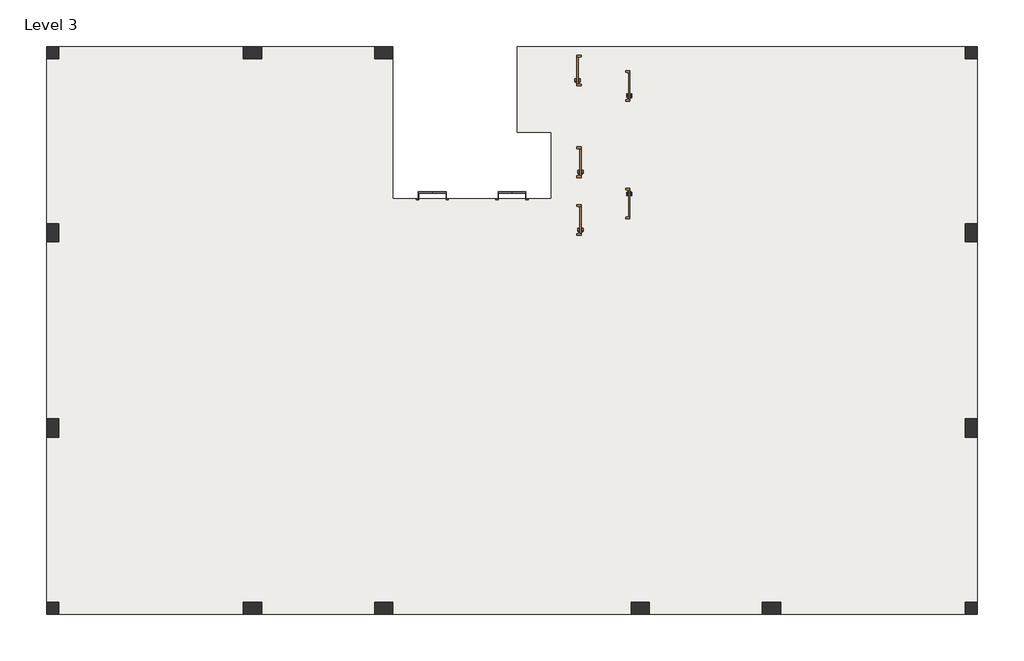
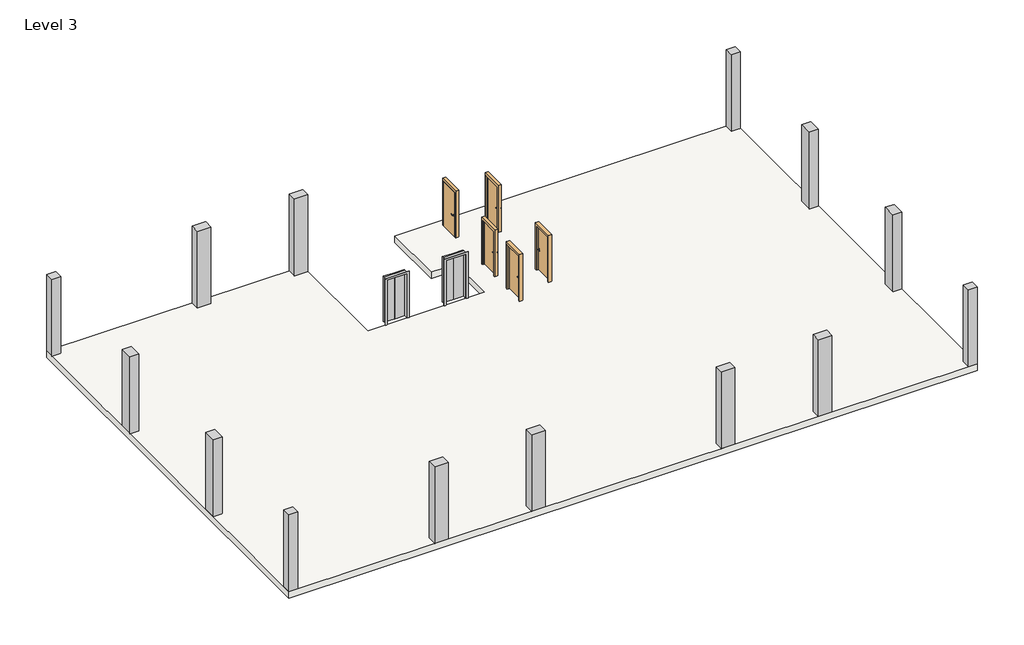
# One storey: 14 columns, 5 doors, 2 proxies, 1 slab.
"""IFC4 building model written with IfcOpenShell, lengths in millimetres."""

import ifcopenshell
import ifcopenshell.guid

model = None  # the IFC model being written
_history = None  # IfcOwnerHistory: only IFC2X3 demands one
_inside = {}  # id of a spatial element -> (the spatial element, [elements in it])
_under = {}  # id of a project, library or spatial element -> (it, [spatial elements below it])
_declared = {}  # id of a project -> (the project, [libraries it declares])
_typed = {}  # id of a type object -> (the type object, [elements of that type])
_made_of = {}  # id of a material, layer set ... -> (it, [elements and type objects made of it])


def new_model(schema):
    """Start an empty IFC model of exactly this schema.

    Asked for "IFC4X3", IfcOpenShell would pick the latest addendum, in which some entities
    have other attributes; the version numbers below select the first issue.
    IFC2X3 requires an IfcOwnerHistory on every rooted entity: one is made here for all.
    """
    global model, _history
    if schema == "IFC4X3":
        model = ifcopenshell.file(schema_version=(4, 3, 0, 0))
    else:
        model = ifcopenshell.file(schema=schema)
    _inside.clear()
    _under.clear()
    _declared.clear()
    _typed.clear()
    _made_of.clear()
    _history = None
    if model.schema == "IFC2X3":
        org = make("IfcOrganization", Name="unknown")
        user = make(
            "IfcPersonAndOrganization",
            ThePerson=make("IfcPerson", FamilyName="unknown"),
            TheOrganization=org,
        )
        app = make(
            "IfcApplication",
            ApplicationDeveloper=org,
            Version="unknown",
            ApplicationFullName="unknown",
            ApplicationIdentifier="unknown",
        )
        _history = make(
            "IfcOwnerHistory",
            OwningUser=user,
            OwningApplication=app,
            ChangeAction="ADDED",
            CreationDate=0,
        )
    return model


def make(cls, **values):
    """One entity of the class cls with the attributes given. An attribute that is None is left unset."""
    return model.create_entity(
        cls, **{name: value for name, value in values.items() if value is not None}
    )


def rooted(cls, **values):
    """An entity with a GlobalId (a new one), such as an element, a storey or a relation."""
    return make(cls, GlobalId=ifcopenshell.guid.new(), OwnerHistory=_history, **values)


def si_unit(unit_type, name, prefix=None):
    """IfcSIUnit, for example si_unit("LENGTHUNIT", "METRE", prefix="MILLI")."""
    return make("IfcSIUnit", UnitType=unit_type, Prefix=prefix, Name=name)


def assignment(units):
    """IfcUnitAssignment: the units of a project."""
    return None if units is None else make("IfcUnitAssignment", Units=units)


def point(xyz):
    """IfcCartesianPoint."""
    return None if xyz is None else make("IfcCartesianPoint", Coordinates=xyz)


def direction(xyz):
    """IfcDirection."""
    return None if xyz is None else make("IfcDirection", DirectionRatios=xyz)


def frame(location, z_axis=None, x_axis=None):
    """IfcAxis2Placement3D, a coordinate frame: its origin and axes. An axis left out is left unset."""
    return make(
        "IfcAxis2Placement3D",
        Location=point(location),
        Axis=direction(z_axis),
        RefDirection=direction(x_axis),
    )


def frame_2d(location, x_axis=None):
    """IfcAxis2Placement2D, a coordinate frame in the plane: its origin and x axis."""
    return make(
        "IfcAxis2Placement2D", Location=point(location), RefDirection=direction(x_axis)
    )


def origin():
    """The frame at (0, 0, 0) with its axes left unset."""
    return frame((0.0, 0.0, 0.0))


def origin_with_axes():
    """The frame at (0, 0, 0) with the z axis (0, 0, 1) and the x axis (1, 0, 0) written out."""
    return frame((0.0, 0.0, 0.0), z_axis=(0.0, 0.0, 1.0), x_axis=(1.0, 0.0, 0.0))


def place(relative_to, where):
    """IfcLocalPlacement: puts the frame where relative to a parent placement (None: the world)."""
    return make(
        "IfcLocalPlacement", PlacementRelTo=relative_to, RelativePlacement=where
    )


def context(
    kind, dimensions, precision=None, world=None, true_north=None, identifier=None
):
    """IfcGeometricRepresentationContext, for example the 3D "Model" context."""
    return make(
        "IfcGeometricRepresentationContext",
        ContextIdentifier=identifier,
        ContextType=kind,
        CoordinateSpaceDimension=dimensions,
        Precision=precision,
        WorldCoordinateSystem=world,
        TrueNorth=true_north,
    )


def project(units=None, contexts=None):
    """IfcProject with its units and contexts."""
    return rooted(
        "IfcProject",
        Name="project",
        RepresentationContexts=contexts,
        UnitsInContext=assignment(units),
    )


def spatial(cls, under=None, at=None, **own):
    """A site, building, storey or space (cls), placed at a placement, below another one or the project."""
    s = rooted(cls, ObjectPlacement=at, **own)
    if under is not None:
        _under.setdefault(under.id(), (under, []))[1].append(s)
    return s


def polyline(points):
    """IfcPolyline through the points."""
    return make("IfcPolyline", Points=[point(p) for p in points])


def circle_curve(where, radius):
    """IfcCircle in the frame where."""
    return make("IfcCircle", Position=where, Radius=radius)


def ellipse_curve(where, semi_axis1, semi_axis2):
    """IfcEllipse in the frame where."""
    return make(
        "IfcEllipse", Position=where, SemiAxis1=semi_axis1, SemiAxis2=semi_axis2
    )


def trimmed(basis, trim1, trim2, sense, master):
    """IfcTrimmedCurve: the piece of a basis curve between two trims."""
    return make(
        "IfcTrimmedCurve",
        BasisCurve=basis,
        Trim1=trim1,
        Trim2=trim2,
        SenseAgreement=sense,
        MasterRepresentation=master,
    )


def segment(curve, same_sense, transition):
    """IfcCompositeCurveSegment."""
    return make(
        "IfcCompositeCurveSegment",
        Transition=transition,
        SameSense=same_sense,
        ParentCurve=curve,
    )


def composite_curve(segments, self_intersect=None):
    """IfcCompositeCurve: segments joined end to end."""
    return make("IfcCompositeCurve", Segments=segments, SelfIntersect=self_intersect)


def outline(outer, holes=None, kind="AREA"):
    """IfcArbitraryClosedProfileDef: a profile drawn as a closed curve; with holes, ...WithVoids."""
    if holes is None:
        return make("IfcArbitraryClosedProfileDef", ProfileType=kind, OuterCurve=outer)
    return make(
        "IfcArbitraryProfileDefWithVoids",
        ProfileType=kind,
        OuterCurve=outer,
        InnerCurves=holes,
    )


def extrude(swept, where, along, depth):
    """IfcExtrudedAreaSolid: the profile swept, set in the frame where, extruded along a direction by depth."""
    return make(
        "IfcExtrudedAreaSolid",
        SweptArea=swept,
        Position=where,
        ExtrudedDirection=direction(along),
        Depth=depth,
    )


def faces_of(points, faces, orient=None, outer=None):
    """IfcFace entities. A face is a list of loops; a loop is a list of indices into points, from 0.

    orient and outer hold one flag for each loop. By default every Orientation is true, the
    first loop of a face is its IfcFaceOuterBound and the others are IfcFaceBound.
    """
    made = []
    for i, loops in enumerate(faces):
        bounds = []
        for j, loop in enumerate(loops):
            is_outer = j == 0 if outer is None else outer[i][j]
            bounds.append(
                make(
                    "IfcFaceOuterBound" if is_outer else "IfcFaceBound",
                    Bound=make("IfcPolyLoop", Polygon=[points[k] for k in loop]),
                    Orientation=True if orient is None else orient[i][j],
                )
            )
        made.append(make("IfcFace", Bounds=bounds))
    return made


def faceted_brep(points, faces, orient=None, outer=None, voids=None):
    """IfcFacetedBrep: a solid bounded by flat faces; with voids (closed shells), ...WithVoids."""
    shared = [point(p) for p in points]
    hull = make("IfcClosedShell", CfsFaces=faces_of(shared, faces, orient, outer))
    if voids is None:
        return make("IfcFacetedBrep", Outer=hull)
    return make(
        "IfcFacetedBrepWithVoids",
        Outer=hull,
        Voids=[
            make(cls, CfsFaces=faces_of(shared, fs, o, b)) for cls, fs, o, b in voids
        ],
    )


def shape(context_of_items, identifier, shape_type, items):
    """IfcShapeRepresentation: the items that make up one representation, for example the "Body"."""
    return make(
        "IfcShapeRepresentation",
        ContextOfItems=context_of_items,
        RepresentationIdentifier=identifier,
        RepresentationType=shape_type,
        Items=items,
    )


def source(mapping_origin, context_of_items, identifier, shape_type, items):
    """IfcRepresentationMap: a shape defined once, which mapped items show again and again."""
    return make(
        "IfcRepresentationMap",
        MappingOrigin=mapping_origin,
        MappedRepresentation=shape(context_of_items, identifier, shape_type, items),
    )


def transform(
    local_origin,
    x_axis=None,
    y_axis=None,
    z_axis=None,
    scale=None,
    scale2=None,
    scale3=None,
    uniform=True,
):
    """IfcCartesianTransformationOperator3D, or its non-uniform kind. x_axis, y_axis, z_axis: its Axis1, 2, 3."""
    if uniform:
        return make(
            "IfcCartesianTransformationOperator3D",
            Axis1=direction(x_axis),
            Axis2=direction(y_axis),
            LocalOrigin=point(local_origin),
            Scale=scale,
            Axis3=direction(z_axis),
        )
    return make(
        "IfcCartesianTransformationOperator3DnonUniform",
        Axis1=direction(x_axis),
        Axis2=direction(y_axis),
        LocalOrigin=point(local_origin),
        Scale=scale,
        Axis3=direction(z_axis),
        Scale2=scale2,
        Scale3=scale3,
    )


def mapped(mapping_source, mapping_target):
    """IfcMappedItem: shows the shape of a source again, moved by a transform."""
    return make(
        "IfcMappedItem", MappingSource=mapping_source, MappingTarget=mapping_target
    )


def made_of(thing, what):
    """Note that an element or type object is made of a material, layer set ...; save() writes the relation."""
    if what is not None:
        _made_of.setdefault(what.id(), (what, []))[1].append(thing)
    return thing


def element(
    cls,
    number,
    at=None,
    inside=None,
    cuts=None,
    type_object=None,
    material=None,
    context=None,
    identifier="Body",
    shape_type=None,
    held_by="IfcProductDefinitionShape",
    body=None,
    shapes=None,
    **own,
):
    """One element of the class cls, such as IfcWall. Its Tag is "e" and its number.

    at: its placement. inside: the storey or other place that contains it. cuts: it is an
    opening in that element (IfcRelVoidsElement). A single representation is given by context,
    identifier, shape_type and body (its items); several are given by shapes. held_by: the class
    of the entity that holds the representations. save() writes the other relations.
    """
    e = rooted(cls, Tag="e%d" % number, ObjectPlacement=at, **own)
    if body is not None:
        shapes = [shape(context, identifier, shape_type, body)]
    if shapes is not None:
        e.Representation = make(held_by, Representations=shapes)
    if inside is not None:
        _inside.setdefault(inside.id(), (inside, []))[1].append(e)
    if cuts is not None:
        rooted(
            "IfcRelVoidsElement", RelatingBuildingElement=cuts, RelatedOpeningElement=e
        )
    if type_object is not None:
        _typed.setdefault(type_object.id(), (type_object, []))[1].append(e)
    return made_of(e, material)


def aggregate(whole, parts):
    """IfcRelAggregates: a whole, such as a stair, and the parts it consists of."""
    return rooted("IfcRelAggregates", RelatingObject=whole, RelatedObjects=parts)


def save(model, path):
    """Write the relations noted so far, then the file.

    IfcRelAggregates (storeys below a building ...), IfcRelContainedInSpatialStructure (elements
    in a storey), IfcRelDefinesByType, IfcRelAssociatesMaterial and IfcRelDeclares: one each for
    every whole, place, type object, material and project.
    """
    for whole, parts in _under.values():
        aggregate(whole, parts)
    for where, things in _inside.values():
        rooted(
            "IfcRelContainedInSpatialStructure",
            RelatedElements=things,
            RelatingStructure=where,
        )
    for kind, things in _typed.values():
        rooted("IfcRelDefinesByType", RelatedObjects=things, RelatingType=kind)
    for what, things in _made_of.values():
        rooted("IfcRelAssociatesMaterial", RelatedObjects=things, RelatingMaterial=what)
    for by, libraries in _declared.values():
        rooted("IfcRelDeclares", RelatingContext=by, RelatedDefinitions=libraries)
    model.write(path)


def plane_surface(at):
    """IfcPlane: the flat surface through the origin of the frame at, square to its z axis."""
    return make("IfcPlane", Position=at)


def cylinder_surface(at, radius):
    """IfcCylindricalSurface: all points at the distance radius from the z axis of the frame at."""
    return make("IfcCylindricalSurface", Position=at, Radius=radius)


def revolved_surface(curve, axis_point, axis_direction):
    """IfcSurfaceOfRevolution: the curve turned about the line through axis_point along axis_direction."""
    return make(
        "IfcSurfaceOfRevolution",
        SweptCurve=make("IfcArbitraryOpenProfileDef", ProfileType="CURVE", Curve=curve),
        AxisPosition=make("IfcAxis1Placement", Location=point(axis_point), Axis=direction(axis_direction)),
    )


def advanced_brep(points, edges, surfaces, faces):
    """IfcAdvancedBrep: a solid bounded by faces that lie on surfaces and meet in shared edges.

    An edge is (start, end): straight between two places in points (the first is 0);
    or (start, end, curve); or (start, end, curve, False) where it runs against its curve.
    A face is (place in surfaces, loops), or (place, loops, False) where it looks against
    its surface's normal. A loop lists edges by number (the first is 1), with a minus sign
    where the edge is run from its end to its start. The first loop is the outer one.
    """
    corners = [point(p) for p in points]
    vertices = [make("IfcVertexPoint", VertexGeometry=c) for c in corners]
    made = []
    for start, end, *more in edges:
        made.append(
            make(
                "IfcEdgeCurve",
                EdgeStart=vertices[start],
                EdgeEnd=vertices[end],
                EdgeGeometry=more[0] if more else make("IfcPolyline", Points=[corners[start], corners[end]]),
                SameSense=more[1] if len(more) > 1 else True,
            )
        )
    hull = []
    for where, loops, *sense in faces:
        bounds = []
        for j, loop in enumerate(loops):
            ring = [make("IfcOrientedEdge", EdgeElement=made[abs(k) - 1], Orientation=k > 0) for k in loop]
            bounds.append(
                make(
                    "IfcFaceOuterBound" if j == 0 else "IfcFaceBound",
                    Bound=make("IfcEdgeLoop", EdgeList=ring),
                    Orientation=True,
                )
            )
        hull.append(make("IfcAdvancedFace", Bounds=bounds, FaceSurface=surfaces[where], SameSense=sense[0] if sense else True))
    return make("IfcAdvancedBrep", Outer=make("IfcClosedShell", CfsFaces=hull))


def proxy_71d7088b(model_context):
    return source(origin(), model_context, "Body", "SweptSolid", [
        extrude(outline(polyline([(-102.3106443, 96.8375), (-562.6856443, 96.8375), (-562.6856443, 147.6375), (-102.3106443, 147.6375), (-102.3106443, 96.8375)])), origin_with_axes(), (0.0, 0.0, 1.0), 2159.0),
        extrude(outline(polyline([(364.4143557, 96.8375), (-95.9606443, 96.8375), (-95.9606443, 147.6375), (364.4143557, 147.6375), (364.4143557, 96.8375)])), origin_with_axes(), (0.0, 0.0, 1.0), 2159.0),
        extrude(outline(polyline([(0.0, -562.6856443), (0.0, -556.3356443), (2133.6, -556.3356443), (2133.6, 358.0643557), (0.0, 358.0643557), (0.0, 364.4143557), (2159.0, 364.4143557), (2159.0, -562.6856443), (0.0, -562.6856443)])), frame((0.0, -96.8375, 0.0), z_axis=(0.0, 1.0, 0.0), x_axis=(0.0, 0.0, 1.0)), (0.0, 0.0, 1.0), 193.675),
        extrude(outline(polyline([(0.0, -632.5356443), (0.0, -556.3356443), (2133.6, -556.3356443), (2133.6, 358.0643557), (0.0, 358.0643557), (0.0, 434.2643557), (2209.8, 434.2643557), (2209.8, -632.5356443), (0.0, -632.5356443)])), frame((0.0, -122.2375, 0.0), z_axis=(0.0, 1.0, 0.0), x_axis=(0.0, 0.0, 1.0)), (0.0, 0.0, 1.0), 25.4),
    ])


def door_9f6fe377(model_context):
    return source(origin(), model_context, "Body", "SolidModel", [
        advanced_brep(
        [(-392.190625, -25.3375, 1016.0), (-372.190625, -25.3375, 1016.0), (-392.190625, 4.6625, 1016.0), (-372.190625, 4.6625, 1016.0), (-367.190625, 9.6625, 1016.0), (-367.190625, 29.6625, 1016.0), (-262.190625, 29.6625, 1016.0), (-262.190625, 9.6625, 1016.0)],
        [
            (0, 1, circle_curve(frame((-382.190625, -25.3375, 1016.0), z_axis=(0.0, -1.0, 0.0), x_axis=(1.0, 0.0, 0.0)), 10.0)),
            (1, 0, circle_curve(frame((-382.190625, -25.3375, 1016.0), z_axis=(0.0, -1.0, 0.0), x_axis=(1.0, 0.0, 0.0)), 10.0)),
            (0, 2),
            (2, 3, circle_curve(frame((-382.190625, 4.6625, 1016.0), z_axis=(0.0, -1.0, 0.0), x_axis=(1.0, 0.0, 0.0)), 10.0)),
            (3, 1),
            (3, 2, circle_curve(frame((-382.190625, 4.6625, 1016.0), z_axis=(0.0, -1.0, 0.0), x_axis=(1.0, 0.0, 0.0)), 10.0)),
            (4, 3, circle_curve(frame((-367.190625, 4.6625, 1016.0), z_axis=(0.0, 0.0, 1.0), x_axis=(-1.0, 0.0, 0.0)), 5.0)),
            (2, 5, circle_curve(frame((-367.190625, 4.6625, 1016.0), z_axis=(0.0, 0.0, -1.0), x_axis=(-1.0, 0.0, 0.0)), 25.0)),
            (5, 4, circle_curve(frame((-367.190625, 19.6625, 1016.0), z_axis=(-1.0, 0.0, 0.0), x_axis=(0.0, -1.0, 0.0)), 10.0)),
            (4, 5, circle_curve(frame((-367.190625, 19.6625, 1016.0), z_axis=(-1.0, 0.0, 0.0), x_axis=(0.0, -1.0, 0.0)), 10.0)),
            (6, 7, circle_curve(frame((-262.190625, 19.6625, 1016.0), z_axis=(1.0, 0.0, 0.0), x_axis=(0.0, -1.0, 0.0)), 10.0)),
            (7, 6, circle_curve(frame((-262.190625, 19.6625, 1016.0), z_axis=(1.0, 0.0, 0.0), x_axis=(0.0, -1.0, 0.0)), 10.0)),
            (5, 6),
            (7, 4),
        ],
        [
            plane_surface(frame((-382.190625, -25.3375, 1016.0), z_axis=(0.0, -1.0, 0.0), x_axis=(0.0, 0.0, 1.0))),
            cylinder_surface(frame((-382.190625, -25.3375, 1016.0), z_axis=(0.0, -1.0, 0.0), x_axis=(1.0, 0.0, 0.0)), 10.0),
            revolved_surface(trimmed(ellipse_curve(frame((-382.190625, 4.6625, 1016.0), z_axis=(0.0, -1.0, 0.0), x_axis=(1.0, 0.0, 0.0)), 10.0, 10.0), [point((-392.190625, 4.6625, 1016.0))], [point((-372.190625, 4.6625, 1016.0))], True, "CARTESIAN"), (-367.190625, 4.6625, 1016.0), (0.0, 0.0, -1.0)),
            revolved_surface(trimmed(ellipse_curve(frame((-382.190625, 4.6625, 1016.0), z_axis=(0.0, -1.0, 0.0), x_axis=(1.0, 0.0, 0.0)), 10.0, 10.0), [point((-372.190625, 4.6625, 1016.0))], [point((-392.190625, 4.6625, 1016.0))], True, "CARTESIAN"), (-367.190625, 4.6625, 1016.0), (0.0, 0.0, -1.0)),
            plane_surface(frame((-262.190625, 19.6625, 1016.0), z_axis=(1.0, 0.0, 0.0), x_axis=(0.0, 0.0, 1.0))),
            cylinder_surface(frame((-367.190625, 19.6625, 1016.0), z_axis=(-1.0, 0.0, 0.0), x_axis=(0.0, -1.0, 0.0)), 10.0),
        ],
        [
            (0, [[1, 2]]),
            (1, [[-1, 3, 4, 5]]),
            (1, [[-2, -5, 6, -3]]),
            (2, [[7, -4, 8, 9]]),
            (3, [[-8, -6, -7, 10]]),
            (4, [[11, 12]]),
            (5, [[-9, 13, -12, 14]]),
            (5, [[-10, -14, -11, -13]]),
        ],
    ),
        extrude(outline(composite_curve([segment(trimmed(circle_curve(frame_2d((1016.0, -384.690625)), 30.0), [point((1016.0, -414.690625))], [point((1016.0, -354.690625))], False, "CARTESIAN"), True, "CONTINUOUS"), segment(trimmed(circle_curve(frame_2d((1016.0, -384.690625)), 30.0), [point((1016.0, -354.690625))], [point((1016.0, -414.690625))], False, "CARTESIAN"), True, "CONTINUOUS")], self_intersect=False)), frame((0.0, -33.3375, 0.0), z_axis=(0.0, 1.0, 0.0), x_axis=(0.0, 0.0, 1.0)), (0.0, 0.0, 1.0), 8.0),
        advanced_brep(
        [(-392.190625, -85.7875, 1016.0), (-372.190625, -85.7875, 1016.0), (-372.190625, -115.7875, 1016.0), (-392.190625, -115.7875, 1016.0), (-367.190625, -120.7875, 1016.0), (-367.190625, -140.7875, 1016.0), (-262.190625, -140.7875, 1016.0), (-262.190625, -120.7875, 1016.0)],
        [
            (0, 1, circle_curve(frame((-382.190625, -85.7875, 1016.0), z_axis=(0.0, 1.0, 0.0), x_axis=(1.0, 0.0, 0.0)), 10.0)),
            (1, 0, circle_curve(frame((-382.190625, -85.7875, 1016.0), z_axis=(0.0, 1.0, 0.0), x_axis=(1.0, 0.0, 0.0)), 10.0)),
            (1, 2),
            (2, 3, circle_curve(frame((-382.190625, -115.7875, 1016.0), z_axis=(0.0, 1.0, 0.0), x_axis=(1.0, 0.0, 0.0)), 10.0)),
            (3, 0),
            (3, 2, circle_curve(frame((-382.190625, -115.7875, 1016.0), z_axis=(0.0, 1.0, 0.0), x_axis=(1.0, 0.0, 0.0)), 10.0)),
            (4, 5, circle_curve(frame((-367.190625, -130.7875, 1016.0), z_axis=(-1.0, 0.0, 0.0), x_axis=(0.0, 1.0, 0.0)), 10.0)),
            (5, 3, circle_curve(frame((-367.190625, -115.7875, 1016.0), z_axis=(0.0, 0.0, -1.0), x_axis=(-1.0, 0.0, 0.0)), 25.0)),
            (2, 4, circle_curve(frame((-367.190625, -115.7875, 1016.0), z_axis=(0.0, 0.0, 1.0), x_axis=(-1.0, 0.0, 0.0)), 5.0)),
            (5, 4, circle_curve(frame((-367.190625, -130.7875, 1016.0), z_axis=(-1.0, 0.0, 0.0), x_axis=(0.0, 1.0, 0.0)), 10.0)),
            (6, 7, circle_curve(frame((-262.190625, -130.7875, 1016.0), z_axis=(1.0, 0.0, 0.0), x_axis=(0.0, 1.0, 0.0)), 10.0)),
            (7, 6, circle_curve(frame((-262.190625, -130.7875, 1016.0), z_axis=(1.0, 0.0, 0.0), x_axis=(0.0, 1.0, 0.0)), 10.0)),
            (4, 7),
            (6, 5),
        ],
        [
            plane_surface(frame((-382.190625, -85.7875, 1016.0), z_axis=(0.0, 1.0, 0.0), x_axis=(0.0, 0.0, 1.0))),
            cylinder_surface(frame((-382.190625, -85.7875, 1016.0), z_axis=(0.0, 1.0, 0.0), x_axis=(1.0, 0.0, 0.0)), 10.0),
            revolved_surface(trimmed(ellipse_curve(frame((-382.190625, -115.7875, 1016.0), z_axis=(0.0, -1.0, 0.0), x_axis=(1.0, 0.0, 0.0)), 10.0, 10.0), [point((-392.190625, -115.7875, 1016.0))], [point((-372.190625, -115.7875, 1016.0))], True, "CARTESIAN"), (-367.190625, -115.7875, 1016.0), (0.0, 0.0, -1.0)),
            revolved_surface(trimmed(ellipse_curve(frame((-382.190625, -115.7875, 1016.0), z_axis=(0.0, -1.0, 0.0), x_axis=(1.0, 0.0, 0.0)), 10.0, 10.0), [point((-372.190625, -115.7875, 1016.0))], [point((-392.190625, -115.7875, 1016.0))], True, "CARTESIAN"), (-367.190625, -115.7875, 1016.0), (0.0, 0.0, -1.0)),
            plane_surface(frame((-262.190625, -130.7875, 1016.0), z_axis=(1.0, 0.0, 0.0), x_axis=(0.0, 0.0, 1.0))),
            cylinder_surface(frame((-367.190625, -130.7875, 1016.0), z_axis=(-1.0, 0.0, 0.0), x_axis=(0.0, 1.0, 0.0)), 10.0),
        ],
        [
            (0, [[1, 2]]),
            (1, [[3, 4, 5, -2]]),
            (1, [[-5, 6, -3, -1]]),
            (2, [[7, 8, -4, 9]]),
            (3, [[10, -9, -6, -8]]),
            (4, [[11, 12]]),
            (5, [[13, -11, 14, -7]]),
            (5, [[-14, -12, -13, -10]]),
        ],
    ),
        extrude(outline(composite_curve([segment(trimmed(circle_curve(frame_2d((1016.0, -384.690625)), 30.0), [point((1016.0, -414.690625))], [point((1016.0, -354.690625))], False, "CARTESIAN"), True, "CONTINUOUS"), segment(trimmed(circle_curve(frame_2d((1016.0, -384.690625)), 30.0), [point((1016.0, -354.690625))], [point((1016.0, -414.690625))], False, "CARTESIAN"), True, "CONTINUOUS")], self_intersect=False)), frame((0.0, -85.7875, 0.0), z_axis=(0.0, 1.0, 0.0), x_axis=(0.0, 0.0, 1.0)), (0.0, 0.0, 1.0), 8.0),
        faceted_brep([(457.2, -28.575, 0.0), (441.325, -28.575, 0.0), (441.325, 19.05, 0.0), (457.2, 19.05, 0.0), (457.2, 68.2625, 0.0), (508.0, 68.2625, 0.0), (508.0, -77.7875, 0.0), (457.2, -77.7875, 0.0), (457.2, -77.7875, 2133.6), (457.2, -28.575, 2133.6), (508.0, -77.7875, 2235.2), (-508.0, -77.7875, 2235.2), (-508.0, -77.7875, 0.0), (-457.2, -77.7875, 0.0), (-457.2, -77.7875, 2133.6), (508.0, 68.2625, 2235.2), (457.2, 68.2625, 2133.6), (-457.2, 68.2625, 2133.6), (-457.2, 68.2625, 0.0), (-508.0, 68.2625, 0.0), (-508.0, 68.2625, 2235.2), (457.2, 19.05, 2133.6), (441.325, 19.05, 2117.725), (-441.325, 19.05, 2117.725), (-441.325, 19.05, 0.0), (-457.2, 19.05, 0.0), (-457.2, 19.05, 2133.6), (441.325, -28.575, 2117.725), (-457.2, -28.575, 2133.6), (-457.2, -28.575, 0.0), (-441.325, -28.575, 0.0), (-441.325, -28.575, 2117.725)], [[[0, 1, 2, 3, 4, 5, 6, 7]], [[7, 8, 9, 0]], [[6, 10, 11, 12, 13, 14, 8, 7]], [[5, 15, 10, 6]], [[4, 16, 17, 18, 19, 20, 15, 5]], [[3, 21, 16, 4]], [[2, 22, 23, 24, 25, 26, 21, 3]], [[1, 27, 22, 2]], [[0, 9, 28, 29, 30, 31, 27, 1]], [[8, 14, 28, 9]], [[16, 21, 26, 17]], [[22, 27, 31, 23]], [[12, 19, 18, 25, 24, 30, 29, 13]], [[13, 29, 28, 14]], [[11, 20, 19, 12]], [[17, 26, 25, 18]], [[23, 31, 30, 24]], [[15, 20, 11, 10]]]),
        extrude(outline(polyline([(457.2, -33.3375), (457.2, -77.7875), (-457.2, -77.7875), (-457.2, -33.3375), (457.2, -33.3375)])), origin_with_axes(), (0.0, 0.0, 1.0), 2133.6),
    ])


def door_87fe937e(model_context):
    return source(origin(), model_context, "Body", "SolidModel", [
        advanced_brep(
        [(-392.190625, 25.3375, 1016.0), (-372.190625, 25.3375, 1016.0), (-372.190625, -4.6625, 1016.0), (-392.190625, -4.6625, 1016.0), (-367.190625, -9.6625, 1016.0), (-367.190625, -29.6625, 1016.0), (-262.190625, -29.6625, 1016.0), (-262.190625, -9.6625, 1016.0)],
        [
            (0, 1, circle_curve(frame((-382.190625, 25.3375, 1016.0), z_axis=(0.0, 1.0, 0.0), x_axis=(1.0, 0.0, 0.0)), 10.0)),
            (1, 0, circle_curve(frame((-382.190625, 25.3375, 1016.0), z_axis=(0.0, 1.0, 0.0), x_axis=(1.0, 0.0, 0.0)), 10.0)),
            (1, 2),
            (2, 3, circle_curve(frame((-382.190625, -4.6625, 1016.0), z_axis=(0.0, 1.0, 0.0), x_axis=(1.0, 0.0, 0.0)), 10.0)),
            (3, 0),
            (3, 2, circle_curve(frame((-382.190625, -4.6625, 1016.0), z_axis=(0.0, 1.0, 0.0), x_axis=(1.0, 0.0, 0.0)), 10.0)),
            (4, 5, circle_curve(frame((-367.190625, -19.6625, 1016.0), z_axis=(-1.0, 0.0, 0.0), x_axis=(0.0, 1.0, 0.0)), 10.0)),
            (5, 3, circle_curve(frame((-367.190625, -4.6625, 1016.0), z_axis=(0.0, 0.0, -1.0), x_axis=(-1.0, 0.0, 0.0)), 25.0)),
            (2, 4, circle_curve(frame((-367.190625, -4.6625, 1016.0), z_axis=(0.0, 0.0, 1.0), x_axis=(-1.0, 0.0, 0.0)), 5.0)),
            (5, 4, circle_curve(frame((-367.190625, -19.6625, 1016.0), z_axis=(-1.0, 0.0, 0.0), x_axis=(0.0, 1.0, 0.0)), 10.0)),
            (6, 7, circle_curve(frame((-262.190625, -19.6625, 1016.0), z_axis=(1.0, 0.0, 0.0), x_axis=(0.0, 1.0, 0.0)), 10.0)),
            (7, 6, circle_curve(frame((-262.190625, -19.6625, 1016.0), z_axis=(1.0, 0.0, 0.0), x_axis=(0.0, 1.0, 0.0)), 10.0)),
            (4, 7),
            (6, 5),
        ],
        [
            plane_surface(frame((-382.190625, 25.3375, 1016.0), z_axis=(0.0, 1.0, 0.0), x_axis=(0.0, 0.0, 1.0))),
            cylinder_surface(frame((-382.190625, 25.3375, 1016.0), z_axis=(0.0, 1.0, 0.0), x_axis=(1.0, 0.0, 0.0)), 10.0),
            revolved_surface(trimmed(ellipse_curve(frame((-382.190625, -4.6625, 1016.0), z_axis=(0.0, -1.0, 0.0), x_axis=(1.0, 0.0, 0.0)), 10.0, 10.0), [point((-392.190625, -4.6625, 1016.0))], [point((-372.190625, -4.6625, 1016.0))], True, "CARTESIAN"), (-367.190625, -4.6625, 1016.0), (0.0, 0.0, -1.0)),
            revolved_surface(trimmed(ellipse_curve(frame((-382.190625, -4.6625, 1016.0), z_axis=(0.0, -1.0, 0.0), x_axis=(1.0, 0.0, 0.0)), 10.0, 10.0), [point((-372.190625, -4.6625, 1016.0))], [point((-392.190625, -4.6625, 1016.0))], True, "CARTESIAN"), (-367.190625, -4.6625, 1016.0), (0.0, 0.0, -1.0)),
            plane_surface(frame((-262.190625, -19.6625, 1016.0), z_axis=(1.0, 0.0, 0.0), x_axis=(0.0, 0.0, 1.0))),
            cylinder_surface(frame((-367.190625, -19.6625, 1016.0), z_axis=(-1.0, 0.0, 0.0), x_axis=(0.0, 1.0, 0.0)), 10.0),
        ],
        [
            (0, [[1, 2]]),
            (1, [[3, 4, 5, -2]]),
            (1, [[-5, 6, -3, -1]]),
            (2, [[7, 8, -4, 9]]),
            (3, [[10, -9, -6, -8]]),
            (4, [[11, 12]]),
            (5, [[13, -11, 14, -7]]),
            (5, [[-14, -12, -13, -10]]),
        ],
    ),
        extrude(outline(composite_curve([segment(trimmed(circle_curve(frame_2d((1016.0, -384.690625)), 30.0), [point((1016.0, -414.690625))], [point((1016.0, -354.690625))], False, "CARTESIAN"), True, "CONTINUOUS"), segment(trimmed(circle_curve(frame_2d((1016.0, -384.690625)), 30.0), [point((1016.0, -354.690625))], [point((1016.0, -414.690625))], False, "CARTESIAN"), True, "CONTINUOUS")], self_intersect=False)), frame((0.0, 25.3375, 0.0), z_axis=(0.0, 1.0, 0.0), x_axis=(0.0, 0.0, 1.0)), (0.0, 0.0, 1.0), 8.0),
        advanced_brep(
        [(-392.190625, 85.7875, 1016.0), (-372.190625, 85.7875, 1016.0), (-392.190625, 115.7875, 1016.0), (-372.190625, 115.7875, 1016.0), (-367.190625, 120.7875, 1016.0), (-367.190625, 140.7875, 1016.0), (-262.190625, 140.7875, 1016.0), (-262.190625, 120.7875, 1016.0)],
        [
            (0, 1, circle_curve(frame((-382.190625, 85.7875, 1016.0), z_axis=(0.0, -1.0, 0.0), x_axis=(1.0, 0.0, 0.0)), 10.0)),
            (1, 0, circle_curve(frame((-382.190625, 85.7875, 1016.0), z_axis=(0.0, -1.0, 0.0), x_axis=(1.0, 0.0, 0.0)), 10.0)),
            (0, 2),
            (2, 3, circle_curve(frame((-382.190625, 115.7875, 1016.0), z_axis=(0.0, -1.0, 0.0), x_axis=(1.0, 0.0, 0.0)), 10.0)),
            (3, 1),
            (3, 2, circle_curve(frame((-382.190625, 115.7875, 1016.0), z_axis=(0.0, -1.0, 0.0), x_axis=(1.0, 0.0, 0.0)), 10.0)),
            (4, 3, circle_curve(frame((-367.190625, 115.7875, 1016.0), z_axis=(0.0, 0.0, 1.0), x_axis=(-1.0, 0.0, 0.0)), 5.0)),
            (2, 5, circle_curve(frame((-367.190625, 115.7875, 1016.0), z_axis=(0.0, 0.0, -1.0), x_axis=(-1.0, 0.0, 0.0)), 25.0)),
            (5, 4, circle_curve(frame((-367.190625, 130.7875, 1016.0), z_axis=(-1.0, 0.0, 0.0), x_axis=(0.0, -1.0, 0.0)), 10.0)),
            (4, 5, circle_curve(frame((-367.190625, 130.7875, 1016.0), z_axis=(-1.0, 0.0, 0.0), x_axis=(0.0, -1.0, 0.0)), 10.0)),
            (6, 7, circle_curve(frame((-262.190625, 130.7875, 1016.0), z_axis=(1.0, 0.0, 0.0), x_axis=(0.0, -1.0, 0.0)), 10.0)),
            (7, 6, circle_curve(frame((-262.190625, 130.7875, 1016.0), z_axis=(1.0, 0.0, 0.0), x_axis=(0.0, -1.0, 0.0)), 10.0)),
            (5, 6),
            (7, 4),
        ],
        [
            plane_surface(frame((-382.190625, 85.7875, 1016.0), z_axis=(0.0, -1.0, 0.0), x_axis=(0.0, 0.0, 1.0))),
            cylinder_surface(frame((-382.190625, 85.7875, 1016.0), z_axis=(0.0, -1.0, 0.0), x_axis=(1.0, 0.0, 0.0)), 10.0),
            revolved_surface(trimmed(ellipse_curve(frame((-382.190625, 115.7875, 1016.0), z_axis=(0.0, -1.0, 0.0), x_axis=(1.0, 0.0, 0.0)), 10.0, 10.0), [point((-392.190625, 115.7875, 1016.0))], [point((-372.190625, 115.7875, 1016.0))], True, "CARTESIAN"), (-367.190625, 115.7875, 1016.0), (0.0, 0.0, -1.0)),
            revolved_surface(trimmed(ellipse_curve(frame((-382.190625, 115.7875, 1016.0), z_axis=(0.0, -1.0, 0.0), x_axis=(1.0, 0.0, 0.0)), 10.0, 10.0), [point((-372.190625, 115.7875, 1016.0))], [point((-392.190625, 115.7875, 1016.0))], True, "CARTESIAN"), (-367.190625, 115.7875, 1016.0), (0.0, 0.0, -1.0)),
            plane_surface(frame((-262.190625, 130.7875, 1016.0), z_axis=(1.0, 0.0, 0.0), x_axis=(0.0, 0.0, 1.0))),
            cylinder_surface(frame((-367.190625, 130.7875, 1016.0), z_axis=(-1.0, 0.0, 0.0), x_axis=(0.0, -1.0, 0.0)), 10.0),
        ],
        [
            (0, [[1, 2]]),
            (1, [[-1, 3, 4, 5]]),
            (1, [[-2, -5, 6, -3]]),
            (2, [[7, -4, 8, 9]]),
            (3, [[-8, -6, -7, 10]]),
            (4, [[11, 12]]),
            (5, [[-9, 13, -12, 14]]),
            (5, [[-10, -14, -11, -13]]),
        ],
    ),
        extrude(outline(composite_curve([segment(trimmed(circle_curve(frame_2d((1016.0, -384.690625)), 30.0), [point((1016.0, -414.690625))], [point((1016.0, -354.690625))], False, "CARTESIAN"), True, "CONTINUOUS"), segment(trimmed(circle_curve(frame_2d((1016.0, -384.690625)), 30.0), [point((1016.0, -354.690625))], [point((1016.0, -414.690625))], False, "CARTESIAN"), True, "CONTINUOUS")], self_intersect=False)), frame((0.0, 77.7875, 0.0), z_axis=(0.0, 1.0, 0.0), x_axis=(0.0, 0.0, 1.0)), (0.0, 0.0, 1.0), 8.0),
        faceted_brep([(457.2, 28.575, 0.0), (457.2, 77.7875, 0.0), (508.0, 77.7875, 0.0), (508.0, -68.2625, 0.0), (457.2, -68.2625, 0.0), (457.2, -19.05, 0.0), (441.325, -19.05, 0.0), (441.325, 28.575, 0.0), (457.2, 28.575, 2133.6), (457.2, 77.7875, 2133.6), (-457.2, 77.7875, 2133.6), (-457.2, 77.7875, 0.0), (-508.0, 77.7875, 0.0), (-508.0, 77.7875, 2235.2), (508.0, 77.7875, 2235.2), (508.0, -68.2625, 2235.2), (-508.0, -68.2625, 2235.2), (-508.0, -68.2625, 0.0), (-457.2, -68.2625, 0.0), (-457.2, -68.2625, 2133.6), (457.2, -68.2625, 2133.6), (457.2, -19.05, 2133.6), (-457.2, -19.05, 2133.6), (-457.2, -19.05, 0.0), (-441.325, -19.05, 0.0), (-441.325, -19.05, 2117.725), (441.325, -19.05, 2117.725), (441.325, 28.575, 2117.725), (-441.325, 28.575, 2117.725), (-441.325, 28.575, 0.0), (-457.2, 28.575, 0.0), (-457.2, 28.575, 2133.6)], [[[0, 1, 2, 3, 4, 5, 6, 7]], [[1, 0, 8, 9]], [[2, 1, 9, 10, 11, 12, 13, 14]], [[3, 2, 14, 15]], [[4, 3, 15, 16, 17, 18, 19, 20]], [[5, 4, 20, 21]], [[6, 5, 21, 22, 23, 24, 25, 26]], [[7, 6, 26, 27]], [[0, 7, 27, 28, 29, 30, 31, 8]], [[9, 8, 31, 10]], [[20, 19, 22, 21]], [[26, 25, 28, 27]], [[12, 11, 30, 29, 24, 23, 18, 17]], [[11, 10, 31, 30]], [[13, 12, 17, 16]], [[19, 18, 23, 22]], [[25, 24, 29, 28]], [[15, 14, 13, 16]]]),
        extrude(outline(polyline([(457.2, 33.3375), (-457.2, 33.3375), (-457.2, 77.7875), (457.2, 77.7875), (457.2, 33.3375)])), origin_with_axes(), (0.0, 0.0, 1.0), 2133.6),
    ])


model = new_model("IFC4")

# Units and contexts
model_context = context("Model", 3, world=origin())
ifc_project = project(units=[si_unit("LENGTHUNIT", "METRE", prefix="MILLI")], contexts=[model_context])

# Site, building, storey
site = spatial("IfcSite", under=ifc_project)
building = spatial("IfcBuilding", under=site)
storey = spatial("IfcBuildingStorey", under=building, Name="Level 3", Elevation=7315.2)

# Proxies
placement = place(None, origin())
proxy_shape = proxy_71d7088b(model_context)
element("IfcBuildingElementProxy", 1, Name="Elevator Door-Center : 36\" x 84\"", ObjectType="Elevator Door-Center : 36\" x 84\"", at=placement, inside=storey, context=model_context, shape_type="MappedRepresentation", body=[
    mapped(proxy_shape, transform((-3717.8016289, 4317.8640304, 7315.2), x_axis=(1.0, 0.0, 0.0), y_axis=(0.0, 1.0, 0.0), z_axis=(0.0, 0.0, 1.0))),
])
element("IfcBuildingElementProxy", 2, Name="Elevator Door-Center : 36\" x 84\"", ObjectType="Elevator Door-Center : 36\" x 84\"", at=placement, inside=storey, context=model_context, shape_type="MappedRepresentation", body=[
    mapped(proxy_shape, transform((-1066.6766289, 4317.8640304, 7315.2), x_axis=(1.0, 0.0, 0.0), y_axis=(0.0, 1.0, 0.0), z_axis=(0.0, 0.0, 1.0))),
])

# Columns
element("IfcColumn", 3, ObjectType="Rectangular Column : 24\" x 24\"", at=placement, inside=storey, context=model_context, shape_type="SweptSolid", body=[
    extrude(outline(polyline([(-16253.4122732, 9291.5015304), (-16253.4122732, 8885.1015304), (-16659.8122732, 8885.1015304), (-16659.8122732, 9291.5015304), (-16253.4122732, 9291.5015304)])), frame((0.0, 0.0, 7315.2), z_axis=(0.0, 0.0, 1.0), x_axis=(1.0, 0.0, 0.0)), (0.0, 0.0, 1.0), 3657.6),
])
element("IfcColumn", 4, ObjectType="Rectangular Column : 24\" x 24\"", at=placement, inside=storey, context=model_context, shape_type="SweptSolid", body=[
    extrude(outline(polyline([(-16253.4122732, 3398.7015304), (-16253.4122732, 2789.1015304), (-16659.8122732, 2789.1015304), (-16659.8122732, 3398.7015304), (-16253.4122732, 3398.7015304)])), frame((0.0, 0.0, 7315.2), z_axis=(0.0, 0.0, 1.0), x_axis=(1.0, 0.0, 0.0)), (0.0, 0.0, 1.0), 3657.6),
])
element("IfcColumn", 5, ObjectType="Rectangular Column : 24\" x 24\"", at=placement, inside=storey, context=model_context, shape_type="SweptSolid", body=[
    extrude(outline(polyline([(-9497.0122732, 8885.1015304), (-10106.6122732, 8885.1015304), (-10106.6122732, 9291.5015304), (-9497.0122732, 9291.5015304), (-9497.0122732, 8885.1015304)])), frame((0.0, 0.0, 7315.2), z_axis=(0.0, 0.0, 1.0), x_axis=(1.0, 0.0, 0.0)), (0.0, 0.0, 1.0), 3657.6),
])
element("IfcColumn", 6, ObjectType="Rectangular Column : 24\" x 24\"", at=placement, inside=storey, context=model_context, shape_type="SweptSolid", body=[
    extrude(outline(polyline([(-5128.2122732, 8885.1015304), (-5737.8122732, 8885.1015304), (-5737.8122732, 9291.5015304), (-5128.2122732, 9291.5015304), (-5128.2122732, 8885.1015304)])), frame((0.0, 0.0, 7315.2), z_axis=(0.0, 0.0, 1.0), x_axis=(1.0, 0.0, 0.0)), (0.0, 0.0, 1.0), 3657.6),
])
element("IfcColumn", 7, ObjectType="Rectangular Column : 24\" x 24\"", at=placement, inside=storey, context=model_context, shape_type="SweptSolid", body=[
    extrude(outline(polyline([(14328.1877268, 8885.1015304), (13921.7877268, 8885.1015304), (13921.7877268, 9291.5015304), (14328.1877268, 9291.5015304), (14328.1877268, 8885.1015304)])), frame((0.0, 0.0, 7315.2), z_axis=(0.0, 0.0, 1.0), x_axis=(1.0, 0.0, 0.0)), (0.0, 0.0, 1.0), 3657.6),
])
element("IfcColumn", 8, ObjectType="Rectangular Column : 24\" x 24\"", at=placement, inside=storey, context=model_context, shape_type="SweptSolid", body=[
    extrude(outline(polyline([(13921.7877268, 2789.1015304), (13921.7877268, 3398.7015304), (14328.1877268, 3398.7015304), (14328.1877268, 2789.1015304), (13921.7877268, 2789.1015304)])), frame((0.0, 0.0, 7315.2), z_axis=(0.0, 0.0, 1.0), x_axis=(1.0, 0.0, 0.0)), (0.0, 0.0, 1.0), 3657.6),
])
element("IfcColumn", 9, ObjectType="Rectangular Column : 24\" x 24\"", at=placement, inside=storey, context=model_context, shape_type="SweptSolid", body=[
    extrude(outline(polyline([(13921.7877268, -3713.2984696), (13921.7877268, -3103.6984696), (14328.1877268, -3103.6984696), (14328.1877268, -3713.2984696), (13921.7877268, -3713.2984696)])), frame((0.0, 0.0, 7315.2), z_axis=(0.0, 0.0, 1.0), x_axis=(1.0, 0.0, 0.0)), (0.0, 0.0, 1.0), 3657.6),
])
element("IfcColumn", 10, ObjectType="Rectangular Column : 24\" x 24\"", at=placement, inside=storey, context=model_context, shape_type="SweptSolid", body=[
    extrude(outline(polyline([(13921.7877268, -9606.0984696), (13921.7877268, -9199.6984696), (14328.1877268, -9199.6984696), (14328.1877268, -9606.0984696), (13921.7877268, -9606.0984696)])), frame((0.0, 0.0, 7315.2), z_axis=(0.0, 0.0, 1.0), x_axis=(1.0, 0.0, 0.0)), (0.0, 0.0, 1.0), 3657.6),
])
element("IfcColumn", 11, ObjectType="Rectangular Column : 24\" x 24\"", at=placement, inside=storey, context=model_context, shape_type="SweptSolid", body=[
    extrude(outline(polyline([(7165.3877268, -9199.6984696), (7774.9877268, -9199.6984696), (7774.9877268, -9606.0984696), (7165.3877268, -9606.0984696), (7165.3877268, -9199.6984696)])), frame((0.0, 0.0, 7315.2), z_axis=(0.0, 0.0, 1.0), x_axis=(1.0, 0.0, 0.0)), (0.0, 0.0, 1.0), 3657.6),
])
element("IfcColumn", 12, ObjectType="Rectangular Column : 24\" x 24\"", at=placement, inside=storey, context=model_context, shape_type="SweptSolid", body=[
    extrude(outline(polyline([(2796.5877268, -9199.6984696), (3406.1877268, -9199.6984696), (3406.1877268, -9606.0984696), (2796.5877268, -9606.0984696), (2796.5877268, -9199.6984696)])), frame((0.0, 0.0, 7315.2), z_axis=(0.0, 0.0, 1.0), x_axis=(1.0, 0.0, 0.0)), (0.0, 0.0, 1.0), 3657.6),
])
element("IfcColumn", 13, ObjectType="Rectangular Column : 24\" x 24\"", at=placement, inside=storey, context=model_context, shape_type="SweptSolid", body=[
    extrude(outline(polyline([(-5737.8122732, -9199.6984696), (-5128.2122732, -9199.6984696), (-5128.2122732, -9606.0984696), (-5737.8122732, -9606.0984696), (-5737.8122732, -9199.6984696)])), frame((0.0, 0.0, 7315.2), z_axis=(0.0, 0.0, 1.0), x_axis=(1.0, 0.0, 0.0)), (0.0, 0.0, 1.0), 3657.6),
])
element("IfcColumn", 14, ObjectType="Rectangular Column : 24\" x 24\"", at=placement, inside=storey, context=model_context, shape_type="SweptSolid", body=[
    extrude(outline(polyline([(-10106.6122732, -9199.6984696), (-9497.0122732, -9199.6984696), (-9497.0122732, -9606.0984696), (-10106.6122732, -9606.0984696), (-10106.6122732, -9199.6984696)])), frame((0.0, 0.0, 7315.2), z_axis=(0.0, 0.0, 1.0), x_axis=(1.0, 0.0, 0.0)), (0.0, 0.0, 1.0), 3657.6),
])
element("IfcColumn", 15, ObjectType="Rectangular Column : 24\" x 24\"", at=placement, inside=storey, context=model_context, shape_type="SweptSolid", body=[
    extrude(outline(polyline([(-16659.8122732, -9199.6984696), (-16253.4122732, -9199.6984696), (-16253.4122732, -9606.0984696), (-16659.8122732, -9606.0984696), (-16659.8122732, -9199.6984696)])), frame((0.0, 0.0, 7315.2), z_axis=(0.0, 0.0, 1.0), x_axis=(1.0, 0.0, 0.0)), (0.0, 0.0, 1.0), 3657.6),
])
element("IfcColumn", 16, ObjectType="Rectangular Column : 24\" x 24\"", at=placement, inside=storey, context=model_context, shape_type="SweptSolid", body=[
    extrude(outline(polyline([(-16253.4122732, -3103.6984696), (-16253.4122732, -3713.2984696), (-16659.8122732, -3713.2984696), (-16659.8122732, -3103.6984696), (-16253.4122732, -3103.6984696)])), frame((0.0, 0.0, 7315.2), z_axis=(0.0, 0.0, 1.0), x_axis=(1.0, 0.0, 0.0)), (0.0, 0.0, 1.0), 3657.6),
])

# Doors
door_shape = door_9f6fe377(model_context)
element("IfcDoor", 17, ObjectType="Door-Passage-Single-Flush : 36\" x 84\"", at=placement, inside=storey, context=model_context, shape_type="MappedRepresentation", body=[
    mapped(door_shape, transform((1058.2752268, 5440.2265304, 7315.2), x_axis=(0.0, 1.0, 0.0), y_axis=(-1.0, 0.0, 0.0), z_axis=(0.0, 0.0, 1.0))),
])
element("IfcDoor", 18, ObjectType="Door-Passage-Single-Flush : 36\" x 84\"", at=placement, inside=storey, context=model_context, shape_type="MappedRepresentation", body=[
    mapped(door_shape, transform((1058.2752268, 3509.8265304, 7315.2), x_axis=(0.0, 1.0, 0.0), y_axis=(-1.0, 0.0, 0.0), z_axis=(0.0, 0.0, 1.0))),
])
element("IfcDoor", 19, ObjectType="Door-Passage-Single-Flush : 36\" x 84\"", at=placement, inside=storey, context=model_context, shape_type="MappedRepresentation", body=[
    mapped(door_shape, transform((2683.8752268, 7980.2265304, 7315.2), x_axis=(0.0, 1.0, 0.0), y_axis=(-1.0, 0.0, 0.0), z_axis=(0.0, 0.0, 1.0))),
])
door_2_shape = door_87fe937e(model_context)
element("IfcDoor", 20, ObjectType="Door-Passage-Single-Flush : 36\" x 84\"", at=placement, inside=storey, context=model_context, shape_type="MappedRepresentation", body=[
    mapped(door_2_shape, transform((1070.9752268, 8488.2265304, 7315.2), x_axis=(0.0, 1.0, 0.0), y_axis=(-1.0, 0.0, 0.0), z_axis=(0.0, 0.0, 1.0))),
])
element("IfcDoor", 21, ObjectType="Door-Passage-Single-Flush : 36\" x 84\"", at=placement, inside=storey, context=model_context, shape_type="MappedRepresentation", body=[
    mapped(door_2_shape, transform((2683.8752268, 4059.1015304, 7315.2), x_axis=(0.0, -1.0, 0.0), y_axis=(1.0, 0.0, 0.0), z_axis=(0.0, 0.0, 1.0))),
])

# Slab
element("IfcSlab", 22, ObjectType="Generic - 12\"", at=placement, inside=storey, context=model_context, shape_type="Brep", body=[
    faceted_brep([(14328.1877268, 9291.5015304, 7010.4), (14328.1877268, -9606.0984696, 7010.4), (-16659.8122732, -9606.0984696, 7010.4), (-16659.8122732, 9291.5015304, 7010.4), (-5128.2122732, 9291.5015304, 7010.4), (-5128.2122732, 4221.0265304, 7010.4), (-4934.5372732, 4221.0265304, 7010.4), (145.4627268, 4221.0265304, 7010.4), (145.4627268, 6446.7015304, 7010.4), (-988.0122732, 6446.7015304, 7010.4), (-988.0122732, 9291.5015304, 7010.4), (967.7877268, 9291.5015304, 7010.4), (1161.4627268, 9291.5015304, 7010.4), (2593.3877268, 9291.5015304, 7010.4), (2787.0627268, 9291.5015304, 7010.4), (8282.9877268, 9291.5015304, 7010.4), (8476.6627268, 9291.5015304, 7010.4), (14328.1877268, -9606.0984696, 7315.2), (14328.1877268, 9291.5015304, 7315.2), (8476.6627268, 9291.5015304, 7315.2), (8282.9877268, 9291.5015304, 7315.2), (2787.0627268, 9291.5015304, 7315.2), (2593.3877268, 9291.5015304, 7315.2), (1161.4627268, 9291.5015304, 7315.2), (967.7877268, 9291.5015304, 7315.2), (-988.0122732, 9291.5015304, 7315.2), (-988.0122732, 6446.7015304, 7315.2), (145.4627268, 6446.7015304, 7315.2), (145.4627268, 4221.0265304, 7315.2), (-4934.5372732, 4221.0265304, 7315.2), (-5128.2122732, 4221.0265304, 7315.2), (-5128.2122732, 9291.5015304, 7315.2), (-16659.8122732, 9291.5015304, 7315.2), (-16659.8122732, -9606.0984696, 7315.2)], [[[0, 1, 2, 3, 4, 5, 6, 7, 8, 9, 10, 11, 12, 13, 14, 15, 16]], [[17, 18, 19, 20, 21, 22, 23, 24, 25, 26, 27, 28, 29, 30, 31, 32, 33]], [[1, 0, 18, 17]], [[2, 1, 17, 33]], [[3, 2, 33, 32]], [[7, 28, 27, 8]], [[30, 5, 4, 31]], [[28, 7, 6, 5, 30, 29]], [[3, 32, 31, 4]], [[18, 0, 16, 15, 14, 13, 12, 11, 10, 25, 24, 23, 22, 21, 20, 19]], [[8, 27, 26, 9]], [[9, 26, 25, 10]]]),
])

save(model, "model.ifc")

# Revit data of these elements
# Type "Elevator Door-Center : 36\" x 84\""
#   Assembly Code = "D1010"
#   Door Height = 7' - 0"
#   Door Width = 3' - 0"
#   Trim Projection = 0' - 1"
#   Trim Width = 0' - 3"
#   Door Finish = Elevator Door
#   Frame Finish = Door - Frame
#   Default Elevation = 0
# Type "Rectangular Column : 24\" x 24\""
#   Assembly Code = "B1010200"
#   Depth = 2' - 0"
#   Offset Base = 0' - 0"
#   Offset Top = 0' - 0"
#   Width = 2' - 0"
#   Material = none
# Type "Door-Passage-Single-Flush : 36\" x 84\""
#   Type Mark = "1"
#   Assembly Code = "B2030200"
#   Analytic Construction = "Wooden"
#   Thickness = 0' - 1 3/4"
#   Thermal Resistance (R) = 2.5876 (h·ft²·°F)/BTU
#   Swing Angle [instance default] = 90.00°
#   Strike Height = 3' - 4"
#   Rough Width [instance default] = 3' - 4"
#   Rough Height [instance default] = 7' - 4"
#   MF Opening Height [instance default] = 0' - 4"
#   MF Opening Width [instance default] = 0' - 4"
#   Inset Calculate [instance default] = 0' - 4"
#   Masonry Inset [instance default] = 0' - 1"
#   Height = 7' - 0"
#   Width = 3' - 0"
#   Heat Transfer Coefficient (U) = 0.3865 BTU/(h·ft²·°F)
#   Masonry Frame Depth = 0' - 5 3/4"
#   Define Thermal Properties by = 1
#   Masonry Frame [instance default] = yes
#   Function = 1
#   Dry Wall Frame [instance default] = no
#   Panel Material = Wood - Birch
#   Frame Material = Metal - Paint Finish - Grey
#   Door Handle Material = Aluminum
#   Visual Light Transmittance = 0
#   Solar Heat Gain Coefficient = 0
#   Wall Closure = (empty or 0)
# Type "Generic - 12\""
#   Assembly Code = "B1010"
#   Function = 0
#   Layers, outside or top first: 1' - 0" no material (function 1)
# Elements 1, 2 (IfcBuildingElementProxy, "Elevator Door-Center : 36\" x 84\"")
#   Phase Created = New Construction
#   Materials on its faces: "Door - Frame", "Elevator Door"
# Elements 3, 4, 5, 6, 7, 8, 9, 10, 11, 12, 13, 14, 15, 16 (IfcColumn, "Rectangular Column : 24\" x 24\"")
#   Phase Created = New Construction
#   Materials on its faces: "Default Wall"
# Elements 17, 18, 19, 20, 21 (IfcDoor, "Door-Passage-Single-Flush : 36\" x 84\"")
#   Swing Angle = 90.00°
#   Rough Width = 3' - 4"
#   Rough Height = 7' - 4"
#   Masonry Inset = 0' - 1"
#   MF Opening Width = 0' - 4"
#   MF Opening Height = 0' - 4"
#   Inset Calculate = 0' - 4"
#   Masonry Frame = yes
#   Dry Wall Frame = no
#   Phase Created = New Construction
#   Materials on its faces: "Aluminum", "Metal - Paint Finish - Grey", "Wood - Birch"
# Element 22 (IfcSlab, "Generic - 12\"")
#   built-in parameter 1001955 = 1.5708 (stored number, unit not read)
#   Height Offset From Level = 0' - 0"
#   Phase Created = New Construction
#   Materials on its faces: "Default Floor"
# Materials
#   "Elevator Door": class "Metal", colour RGB 57 57 57, transparency 0
#   "Door - Frame": class "Miscellaneous", colour RGB 118 70 51, transparency 0, Cost = 0
#   "Wood - Birch": class "Wood", colour RGB 166 116 52, transparency 0, Cost = 0
#   "Metal - Paint Finish - Grey": class "Paint", colour RGB 104 104 104, transparency 0, Cost = 0
#   "Aluminum": class "Metal", colour RGB 247 247 247, transparency 0, Description = "Aluminum 6061", Cost = 0
#   "Default Wall": class "Miscellaneous", colour RGB 128 128 128, transparency 0, Cost = 0
#   "Default Floor": class "Miscellaneous", colour RGB 128 128 128, transparency 0, Cost = 0
